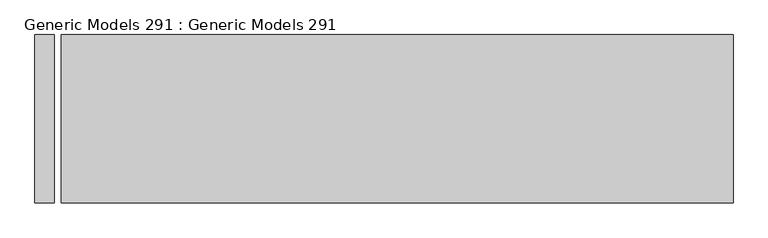
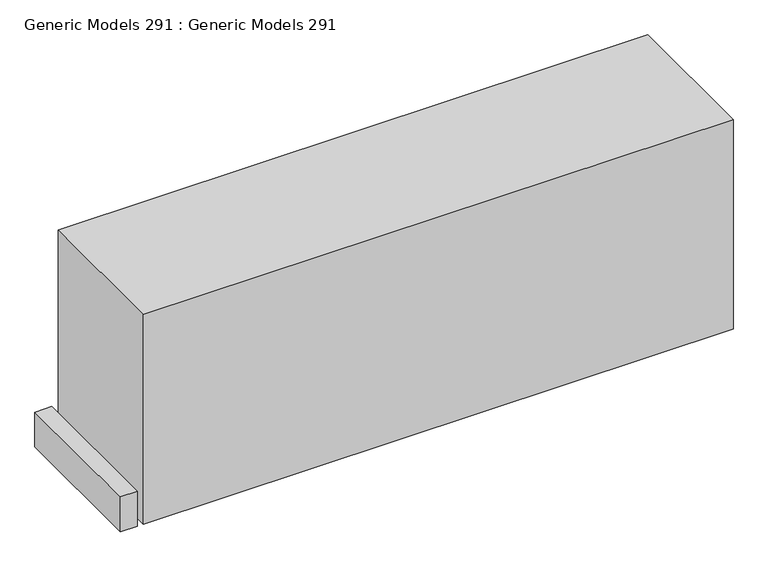
"""IFC4 building model written with IfcOpenShell, lengths in millimetres: proxy geometry, Generic Models 291 : Generic Models 291."""

from ifc_helpers import new_model, si_unit, frame, origin, place, context, project, spatial, polyline, outline, extrude, source, transform, mapped, element, save


def generic_models_291_generic_models_291_3720f25b(model_context):
    return source(origin(), model_context, "Body", "SweptSolid", [
        extrude(outline(polyline([(7162.6263704, 8214.8672747), (7127.6193567, 8214.8672747), (7127.6193567, 8519.6672747), (7162.6263704, 8519.6672747), (7162.6263704, 8214.8672747)])), frame((0.0, 0.0, 123297.696), z_axis=(0.0, 0.0, 1.0), x_axis=(1.0, 0.0, 0.0)), (0.0, 0.0, 1.0), 76.2),
        extrude(outline(polyline([(8392.3149643, 8214.8672747), (7175.3263704, 8214.8672747), (7175.3263704, 8519.6672747), (8392.3149643, 8519.6672747), (8392.3149643, 8214.8672747)])), frame((0.0, 0.0, 123297.696), z_axis=(0.0, 0.0, 1.0), x_axis=(1.0, 0.0, 0.0)), (0.0, 0.0, 1.0), 457.2),
    ])


if __name__ == "__main__":
    model = new_model("IFC4")
    model_context = context("Model", 3, world=origin())
    ifc_project = project(units=[si_unit("LENGTHUNIT", "METRE", prefix="MILLI")], contexts=[model_context])
    site = spatial("IfcSite", under=ifc_project)
    building = spatial("IfcBuilding", under=site)
    placement = place(None, origin())
    generic_models_291_generic_models_291_shape = generic_models_291_generic_models_291_3720f25b(model_context)
    element("IfcBuildingElementProxy", 1, Name="Generic Models 291 : Generic Models 291", ObjectType="Generic Models 291 : Generic Models 291", at=placement, inside=building, context=model_context, shape_type="MappedRepresentation", body=[
        mapped(generic_models_291_generic_models_291_shape, transform((0.0, 0.0, 0.0), x_axis=(1.0, 0.0, 0.0), y_axis=(0.0, 1.0, 0.0), z_axis=(0.0, 0.0, 1.0))),
    ])
    save(model, "model.ifc")

# Revit data of these elements
# Element 1 (IfcBuildingElementProxy, "Generic Models 291 : Generic Models 291")
#   Materials on its faces: "_CONCRETE SLAB W/ WIRE MESH (SEE STRUCT. DWGS) - SLOPE 1% AWAY FROM BUILDING"
# Materials
#   "_CONCRETE SLAB W/ WIRE MESH (SEE STRUCT. DWGS) - SLOPE 1% AWAY FROM BUILDING": class "Generic", colour RGB 191 191 191, transparency 0, Cost = 0
